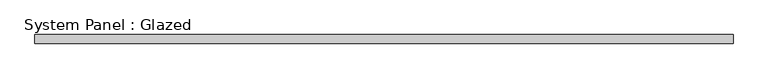
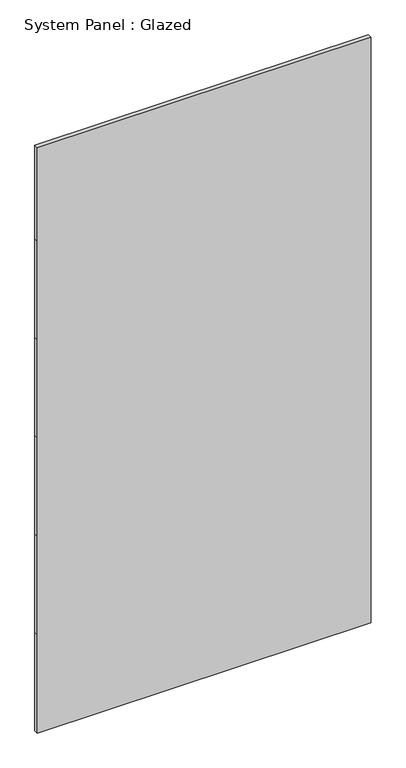
"""IFC4 building model written with IfcOpenShell, lengths in millimetres: plate geometry, System Panel : Glazed."""

import ifcopenshell
import ifcopenshell.guid

model = None  # the IFC model being written
_history = None  # IfcOwnerHistory: only IFC2X3 demands one
_inside = {}  # id of a spatial element -> (the spatial element, [elements in it])
_under = {}  # id of a project, library or spatial element -> (it, [spatial elements below it])
_declared = {}  # id of a project -> (the project, [libraries it declares])
_typed = {}  # id of a type object -> (the type object, [elements of that type])
_made_of = {}  # id of a material, layer set ... -> (it, [elements and type objects made of it])


def new_model(schema):
    """Start an empty IFC model of exactly this schema.

    Asked for "IFC4X3", IfcOpenShell would pick the latest addendum, in which some entities
    have other attributes; the version numbers below select the first issue.
    IFC2X3 requires an IfcOwnerHistory on every rooted entity: one is made here for all.
    """
    global model, _history
    if schema == "IFC4X3":
        model = ifcopenshell.file(schema_version=(4, 3, 0, 0))
    else:
        model = ifcopenshell.file(schema=schema)
    _inside.clear()
    _under.clear()
    _declared.clear()
    _typed.clear()
    _made_of.clear()
    _history = None
    if model.schema == "IFC2X3":
        org = make("IfcOrganization", Name="unknown")
        user = make(
            "IfcPersonAndOrganization",
            ThePerson=make("IfcPerson", FamilyName="unknown"),
            TheOrganization=org,
        )
        app = make(
            "IfcApplication",
            ApplicationDeveloper=org,
            Version="unknown",
            ApplicationFullName="unknown",
            ApplicationIdentifier="unknown",
        )
        _history = make(
            "IfcOwnerHistory",
            OwningUser=user,
            OwningApplication=app,
            ChangeAction="ADDED",
            CreationDate=0,
        )
    return model


def make(cls, **values):
    """One entity of the class cls with the attributes given. An attribute that is None is left unset."""
    return model.create_entity(
        cls, **{name: value for name, value in values.items() if value is not None}
    )


def rooted(cls, **values):
    """An entity with a GlobalId (a new one), such as an element, a storey or a relation."""
    return make(cls, GlobalId=ifcopenshell.guid.new(), OwnerHistory=_history, **values)


def si_unit(unit_type, name, prefix=None):
    """IfcSIUnit, for example si_unit("LENGTHUNIT", "METRE", prefix="MILLI")."""
    return make("IfcSIUnit", UnitType=unit_type, Prefix=prefix, Name=name)


def assignment(units):
    """IfcUnitAssignment: the units of a project."""
    return None if units is None else make("IfcUnitAssignment", Units=units)


def point(xyz):
    """IfcCartesianPoint."""
    return None if xyz is None else make("IfcCartesianPoint", Coordinates=xyz)


def direction(xyz):
    """IfcDirection."""
    return None if xyz is None else make("IfcDirection", DirectionRatios=xyz)


def frame(location, z_axis=None, x_axis=None):
    """IfcAxis2Placement3D, a coordinate frame: its origin and axes. An axis left out is left unset."""
    return make(
        "IfcAxis2Placement3D",
        Location=point(location),
        Axis=direction(z_axis),
        RefDirection=direction(x_axis),
    )


def origin():
    """The frame at (0, 0, 0) with its axes left unset."""
    return frame((0.0, 0.0, 0.0))


def place(relative_to, where):
    """IfcLocalPlacement: puts the frame where relative to a parent placement (None: the world)."""
    return make(
        "IfcLocalPlacement", PlacementRelTo=relative_to, RelativePlacement=where
    )


def context(
    kind, dimensions, precision=None, world=None, true_north=None, identifier=None
):
    """IfcGeometricRepresentationContext, for example the 3D "Model" context."""
    return make(
        "IfcGeometricRepresentationContext",
        ContextIdentifier=identifier,
        ContextType=kind,
        CoordinateSpaceDimension=dimensions,
        Precision=precision,
        WorldCoordinateSystem=world,
        TrueNorth=true_north,
    )


def project(units=None, contexts=None):
    """IfcProject with its units and contexts."""
    return rooted(
        "IfcProject",
        Name="project",
        RepresentationContexts=contexts,
        UnitsInContext=assignment(units),
    )


def spatial(cls, under=None, at=None, **own):
    """A site, building, storey or space (cls), placed at a placement, below another one or the project."""
    s = rooted(cls, ObjectPlacement=at, **own)
    if under is not None:
        _under.setdefault(under.id(), (under, []))[1].append(s)
    return s


def polyline(points):
    """IfcPolyline through the points."""
    return make("IfcPolyline", Points=[point(p) for p in points])


def outline(outer, holes=None, kind="AREA"):
    """IfcArbitraryClosedProfileDef: a profile drawn as a closed curve; with holes, ...WithVoids."""
    if holes is None:
        return make("IfcArbitraryClosedProfileDef", ProfileType=kind, OuterCurve=outer)
    return make(
        "IfcArbitraryProfileDefWithVoids",
        ProfileType=kind,
        OuterCurve=outer,
        InnerCurves=holes,
    )


def extrude(swept, where, along, depth):
    """IfcExtrudedAreaSolid: the profile swept, set in the frame where, extruded along a direction by depth."""
    return make(
        "IfcExtrudedAreaSolid",
        SweptArea=swept,
        Position=where,
        ExtrudedDirection=direction(along),
        Depth=depth,
    )


def shape(context_of_items, identifier, shape_type, items):
    """IfcShapeRepresentation: the items that make up one representation, for example the "Body"."""
    return make(
        "IfcShapeRepresentation",
        ContextOfItems=context_of_items,
        RepresentationIdentifier=identifier,
        RepresentationType=shape_type,
        Items=items,
    )


def source(mapping_origin, context_of_items, identifier, shape_type, items):
    """IfcRepresentationMap: a shape defined once, which mapped items show again and again."""
    return make(
        "IfcRepresentationMap",
        MappingOrigin=mapping_origin,
        MappedRepresentation=shape(context_of_items, identifier, shape_type, items),
    )


def transform(
    local_origin,
    x_axis=None,
    y_axis=None,
    z_axis=None,
    scale=None,
    scale2=None,
    scale3=None,
    uniform=True,
):
    """IfcCartesianTransformationOperator3D, or its non-uniform kind. x_axis, y_axis, z_axis: its Axis1, 2, 3."""
    if uniform:
        return make(
            "IfcCartesianTransformationOperator3D",
            Axis1=direction(x_axis),
            Axis2=direction(y_axis),
            LocalOrigin=point(local_origin),
            Scale=scale,
            Axis3=direction(z_axis),
        )
    return make(
        "IfcCartesianTransformationOperator3DnonUniform",
        Axis1=direction(x_axis),
        Axis2=direction(y_axis),
        LocalOrigin=point(local_origin),
        Scale=scale,
        Axis3=direction(z_axis),
        Scale2=scale2,
        Scale3=scale3,
    )


def mapped(mapping_source, mapping_target):
    """IfcMappedItem: shows the shape of a source again, moved by a transform."""
    return make(
        "IfcMappedItem", MappingSource=mapping_source, MappingTarget=mapping_target
    )


def made_of(thing, what):
    """Note that an element or type object is made of a material, layer set ...; save() writes the relation."""
    if what is not None:
        _made_of.setdefault(what.id(), (what, []))[1].append(thing)
    return thing


def element(
    cls,
    number,
    at=None,
    inside=None,
    cuts=None,
    type_object=None,
    material=None,
    context=None,
    identifier="Body",
    shape_type=None,
    held_by="IfcProductDefinitionShape",
    body=None,
    shapes=None,
    **own,
):
    """One element of the class cls, such as IfcWall. Its Tag is "e" and its number.

    at: its placement. inside: the storey or other place that contains it. cuts: it is an
    opening in that element (IfcRelVoidsElement). A single representation is given by context,
    identifier, shape_type and body (its items); several are given by shapes. held_by: the class
    of the entity that holds the representations. save() writes the other relations.
    """
    e = rooted(cls, Tag="e%d" % number, ObjectPlacement=at, **own)
    if body is not None:
        shapes = [shape(context, identifier, shape_type, body)]
    if shapes is not None:
        e.Representation = make(held_by, Representations=shapes)
    if inside is not None:
        _inside.setdefault(inside.id(), (inside, []))[1].append(e)
    if cuts is not None:
        rooted(
            "IfcRelVoidsElement", RelatingBuildingElement=cuts, RelatedOpeningElement=e
        )
    if type_object is not None:
        _typed.setdefault(type_object.id(), (type_object, []))[1].append(e)
    return made_of(e, material)


def aggregate(whole, parts):
    """IfcRelAggregates: a whole, such as a stair, and the parts it consists of."""
    return rooted("IfcRelAggregates", RelatingObject=whole, RelatedObjects=parts)


def save(model, path):
    """Write the relations noted so far, then the file.

    IfcRelAggregates (storeys below a building ...), IfcRelContainedInSpatialStructure (elements
    in a storey), IfcRelDefinesByType, IfcRelAssociatesMaterial and IfcRelDeclares: one each for
    every whole, place, type object, material and project.
    """
    for whole, parts in _under.values():
        aggregate(whole, parts)
    for where, things in _inside.values():
        rooted(
            "IfcRelContainedInSpatialStructure",
            RelatedElements=things,
            RelatingStructure=where,
        )
    for kind, things in _typed.values():
        rooted("IfcRelDefinesByType", RelatedObjects=things, RelatingType=kind)
    for what, things in _made_of.values():
        rooted("IfcRelAssociatesMaterial", RelatedObjects=things, RelatingMaterial=what)
    for by, libraries in _declared.values():
        rooted("IfcRelDeclares", RelatingContext=by, RelatedDefinitions=libraries)
    model.write(path)


def system_panel_glazed_28c22e26(model_context):
    return source(origin(), model_context, "Body", "SweptSolid", [
        extrude(outline(polyline([(0.0, -977.9), (0.0, 977.9), (609.6, 977.9), (1219.2, 977.9), (1828.8, 977.9), (2438.4, 977.9), (3048.0, 977.9), (3625.85, 977.9), (3625.85, -977.9), (3048.0, -977.9), (2438.4, -977.9), (1828.8, -977.9), (1219.2, -977.9), (609.6, -977.9), (0.0, -977.9)])), frame((0.0, 19.05, 0.0), z_axis=(0.0, 1.0, 0.0), x_axis=(0.0, 0.0, 1.0)), (0.0, 0.0, 1.0), 25.4),
    ])


if __name__ == "__main__":
    model = new_model("IFC4")
    model_context = context("Model", 3, world=origin())
    ifc_project = project(units=[si_unit("LENGTHUNIT", "METRE", prefix="MILLI")], contexts=[model_context])
    site = spatial("IfcSite", under=ifc_project)
    building = spatial("IfcBuilding", under=site)
    placement = place(None, origin())
    system_panel_glazed_shape = system_panel_glazed_28c22e26(model_context)
    element("IfcPlate", 1, ObjectType="System Panel : Glazed", at=placement, inside=building, context=model_context, shape_type="MappedRepresentation", body=[
        mapped(system_panel_glazed_shape, transform((0.0, 0.0, 0.0), x_axis=(1.0, 0.0, 0.0), y_axis=(0.0, 1.0, 0.0), z_axis=(0.0, 0.0, 1.0))),
    ])
    save(model, "model.ifc")

# Revit data of these elements
# Element 1 (IfcPlate, "System Panel : Glazed")
#   Materials on its faces: "Glass"
# Materials
#   "Glass": class "Unassigned", colour RGB 0 0 255, transparency 0.75
